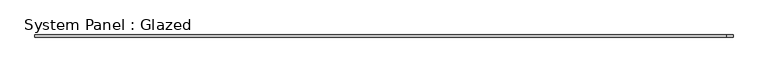
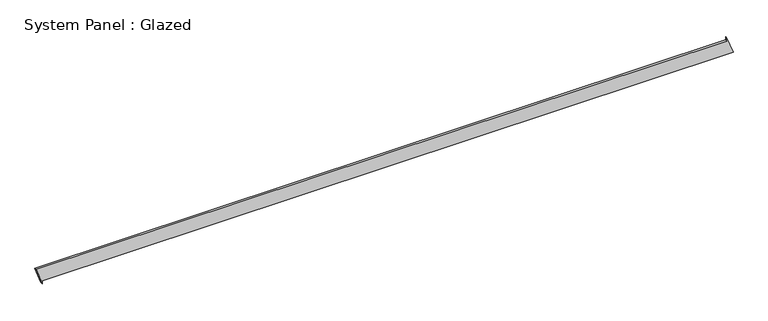
"""IFC4 building model written with IfcOpenShell, lengths in millimetres: plate geometry, System Panel : Glazed."""

from ifc_helpers import new_model, si_unit, frame, origin, place, context, project, spatial, polyline, outline, extrude, source, transform, mapped, element, save


def system_panel_glazed_eac3060f(model_context):
    return source(origin(), model_context, "Body", "SweptSolid", [
        extrude(outline(polyline([(0.0, -3956.878339), (35.3553391, -3956.878339), (35.3553391, 4027.1816216), (233.9801319, 3956.6725023), (198.6247928, 3956.6721138), (198.7125272, -4027.1816216), (0.0, -3956.878339)])), frame((0.0, -49.5, 0.0), z_axis=(0.0, 1.0, 0.0), x_axis=(0.0, 0.0, 1.0)), (0.0, 0.0, 1.0), 25.0),
    ])


if __name__ == "__main__":
    model = new_model("IFC4")
    model_context = context("Model", 3, world=origin())
    ifc_project = project(units=[si_unit("LENGTHUNIT", "METRE", prefix="MILLI")], contexts=[model_context])
    site = spatial("IfcSite", under=ifc_project)
    building = spatial("IfcBuilding", under=site)
    placement = place(None, origin())
    system_panel_glazed_shape = system_panel_glazed_eac3060f(model_context)
    element("IfcPlate", 1, ObjectType="System Panel : Glazed", at=placement, inside=building, context=model_context, shape_type="MappedRepresentation", body=[
        mapped(system_panel_glazed_shape, transform((0.0, 0.0, 0.0), x_axis=(1.0, 0.0, 0.0), y_axis=(0.0, 1.0, 0.0), z_axis=(0.0, 0.0, 1.0))),
    ])
    save(model, "model.ifc")

# Revit data of these elements
# Element 1 (IfcPlate, "System Panel : Glazed")
#   Materials on its faces: "Glass"
# Materials
#   "Glass": class "Glass", colour RGB 218 227 224, transparency 0.85, Description = "Soda Lime Glass", Cost = 0
